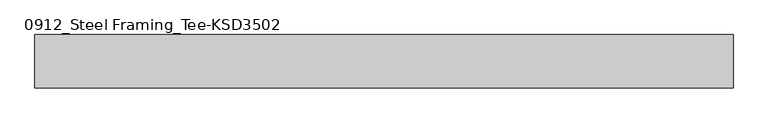
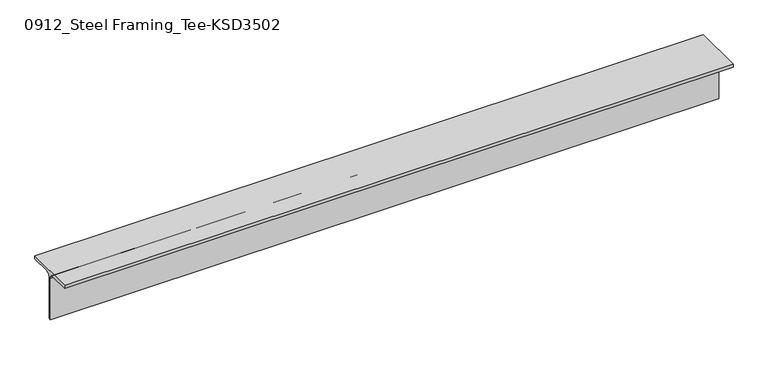
"""IFC4 building model written with IfcOpenShell, lengths in millimetres: member geometry, 0912_Steel Framing_Tee-KSD3502 : H_SB_ASB_CT-150x150x6.5x9."""

from ifc_helpers import new_model, si_unit, point, frame, frame_2d, origin, place, context, project, spatial, polyline, circle_curve, trimmed, segment, composite_curve, outline, extrude, source, transform, mapped, element, save


def member_0912_steel_framing_tee_ksd3502_f18e1055(model_context):
    return source(origin(), model_context, "Body", "SweptSolid", [
        extrude(outline(composite_curve([segment(polyline([(-75.0, 75.0), (75.0, 75.0), (75.0, 66.0), (16.25, 66.0)]), True, "CONTINUOUS"), segment(trimmed(circle_curve(frame_2d((16.25, 53.0)), 13.0), [point((16.25, 66.0))], [point((3.25, 53.0))], True, "CARTESIAN"), True, "CONTINUOUS"), segment(polyline([(3.25, 53.0), (3.25, -75.0), (-3.25, -75.0), (-3.25, 53.0)]), True, "CONTINUOUS"), segment(trimmed(circle_curve(frame_2d((-16.25, 53.0)), 13.0), [point((-3.25, 53.0))], [point((-16.25, 66.0))], True, "CARTESIAN"), True, "CONTINUOUS"), segment(polyline([(-16.25, 66.0), (-75.0, 66.0), (-75.0, 75.0)]), True, "CONTINUOUS")], self_intersect=False)), frame((-1113.65, 0.0, 0.0), z_axis=(1.0, 0.0, 0.0), x_axis=(0.0, 1.0, 0.0)), (0.0, 0.0, 1.0), 1955.9),
    ])


if __name__ == "__main__":
    model = new_model("IFC4")
    model_context = context("Model", 3, world=origin())
    ifc_project = project(units=[si_unit("LENGTHUNIT", "METRE", prefix="MILLI")], contexts=[model_context])
    site = spatial("IfcSite", under=ifc_project)
    building = spatial("IfcBuilding", under=site)
    placement = place(None, origin())
    member_0912_steel_framing_tee_ksd3502_shape = member_0912_steel_framing_tee_ksd3502_f18e1055(model_context)
    element("IfcMember", 1, ObjectType="0912_Steel Framing_Tee-KSD3502 : H_SB_ASB_CT-150x150x6.5x9", at=placement, inside=building, context=model_context, shape_type="MappedRepresentation", body=[
        mapped(member_0912_steel_framing_tee_ksd3502_shape, transform((0.0, 0.0, 0.0), x_axis=(1.0, 0.0, 0.0), y_axis=(0.0, 1.0, 0.0), z_axis=(0.0, 0.0, 1.0))),
    ])
    save(model, "model.ifc")

# Revit data of these elements
# Type "0912_Steel Framing_Tee-KSD3502 : H_SB_ASB_CT-150x150x6.5x9"
#   H_WM Code_1 = "S01AA003-00001 | Main Steel Structure Fabrication Work | Shelter/Building | Light Steel - Standard (30KG/M>Weight) | Material: (   )"
#   H_WM Code_2 = "S03AA029-00001 | Main Steel Structure Erection Work | Shelter/Building | Light Steel (30KG/M>Weight) | Material: (   )"
#   H_WM Code_3 = "S01AA010-00001 | Main Steel Structure Fabrication Work | Shelter/Building | Steel Painting/Coating | for Non-Fireproofed Steel Surface, Surface Preparation, Primer, Second & Final Coat | Material: (   )"
#   H_Q'ty Cal Type Tag = "SB-Q2"
#   Width = 15.0 cm
#   Web Thickness = 0.65 cm
#   Web Fillet = 1.3 cm
#   Section Area = 23.39 cm²
#   Perimeter = 0.60 m²/m
#   Nominal Weight = 18.40 kgf/m
#   Height = 15.0 cm
#   Flange Thickness = 0.9 cm
#   Centroid Vertical = 7.5 cm
#   Centroid Horizontal = 7.5 cm
#   Length [instance default] = 1.5000 m
#   Structural Material [instance default] = Steel, 45-345
#   Warping Constant = (empty or 0)
#   Torsional Moment of Inertia = 0
#   Section Name Key = ""
#   Plastic Modulus weak axis = 0
#   Plastic Modulus strong axis = 0
#   Moment of Inertia weak axis = 0
#   Moment of Inertia strong axis = 0
#   Elastic Modulus weak axis = 0
#   Elastic Modulus strong axis = 0
#   Bolt Spacing = 0
#   Assembly Code = ""
# Element 1 (IfcMember, "0912_Steel Framing_Tee-KSD3502 : H_SB_ASB_CT-150x150x6.5x9")
#   Structural Material = none
# Materials
#   "Steel, 45-345": class "Metal", colour RGB 189 187 185, transparency 0, Description = "Steel 345 MPa", Cost = 0
